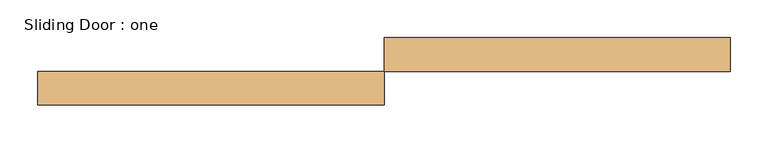
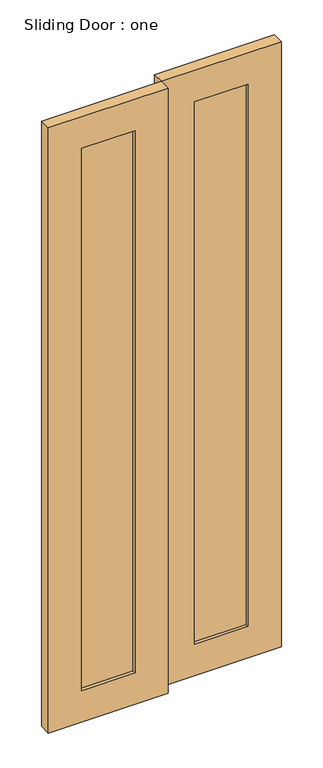
"""IFC4 building model written with IfcOpenShell, lengths in millimetres: door geometry, Sliding Door : one."""

from ifc_helpers import new_model, si_unit, frame, origin, place, context, project, spatial, polyline, outline, extrude, source, transform, mapped, element, save


def sliding_door_one_cf7842af(model_context):
    return source(origin(), model_context, "Body", "SweptSolid", [
        extrude(outline(polyline([(-127.0, -50.8), (-330.2, -50.8), (-330.2, -31.75), (-127.0, -31.75), (-127.0, -50.8)])), frame((0.0, 0.0, 127.0), z_axis=(0.0, 0.0, 1.0), x_axis=(1.0, 0.0, 0.0)), (0.0, 0.0, 1.0), 2184.4),
        extrude(outline(polyline([(330.2, -6.35), (127.0, -6.35), (127.0, 12.7), (330.2, 12.7), (330.2, -6.35)])), frame((0.0, 0.0, 127.0), z_axis=(0.0, 0.0, 1.0), x_axis=(1.0, 0.0, 0.0)), (0.0, 0.0, 1.0), 2184.4),
        extrude(outline(polyline([(2438.4, -457.2), (0.0, -457.2), (0.0, 0.0), (2438.4, 0.0), (2438.4, -457.2)]), holes=[polyline([(127.0, -127.0), (127.0, -330.2), (2311.4, -330.2), (2311.4, -127.0), (127.0, -127.0)])]), frame((0.0, -63.5, 0.0), z_axis=(0.0, 1.0, 0.0), x_axis=(0.0, 0.0, 1.0)), (0.0, 0.0, 1.0), 44.45),
        extrude(outline(polyline([(2438.4, 0.0), (0.0, 0.0), (0.0, 457.2), (2438.4, 457.2), (2438.4, 0.0)]), holes=[polyline([(127.0, 330.2), (127.0, 127.0), (2311.4, 127.0), (2311.4, 330.2), (127.0, 330.2)])]), frame((0.0, -19.05, 0.0), z_axis=(0.0, 1.0, 0.0), x_axis=(0.0, 0.0, 1.0)), (0.0, 0.0, 1.0), 44.45),
    ])


if __name__ == "__main__":
    model = new_model("IFC4")
    model_context = context("Model", 3, world=origin())
    ifc_project = project(units=[si_unit("LENGTHUNIT", "METRE", prefix="MILLI")], contexts=[model_context])
    site = spatial("IfcSite", under=ifc_project)
    building = spatial("IfcBuilding", under=site)
    placement = place(None, origin())
    sliding_door_one_shape = sliding_door_one_cf7842af(model_context)
    element("IfcDoor", 1, ObjectType="Sliding Door : one", at=placement, inside=building, context=model_context, shape_type="MappedRepresentation", body=[
        mapped(sliding_door_one_shape, transform((0.0, 0.0, 0.0), x_axis=(1.0, 0.0, 0.0), y_axis=(0.0, 1.0, 0.0), z_axis=(0.0, 0.0, 1.0))),
    ])
    save(model, "model.ifc")

# Revit data of these elements
# Type "Sliding Door : one"
#   Type Mark = "42"
#   Analytic Construction = "<None>"
#   Stile_Width = 0' - 5"
#   Door_Thickness = 0' - 1 3/4"
#   Door_Offset = 0' - 1"
#   Glass_Material = SAFETY GLAZING
#   Frame_Material = INTERIOR GRADE ALUMINUM STOREFRONT W/ SAFETY GLAZING
#   Function = (empty or 0)
# Element 1 (IfcDoor, "Sliding Door : one")
#   Materials on its faces: "INTERIOR GRADE ALUMINUM STOREFRONT W/ SAFETY GLAZING", "SAFETY GLAZING"
# Materials
#   "SAFETY GLAZING": class "Glass", colour RGB 142 168 196, transparency 0.75, Description = "Soda Lime Glass", Cost = 0
#   "INTERIOR GRADE ALUMINUM STOREFRONT W/ SAFETY GLAZING": class "Metal", colour RGB 226 226 226, transparency 0, Description = "Aluminum 6061", Cost = 0
